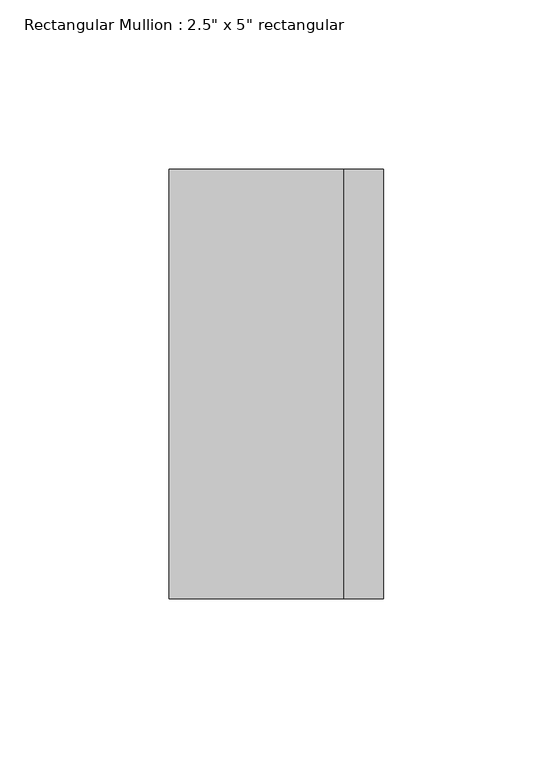
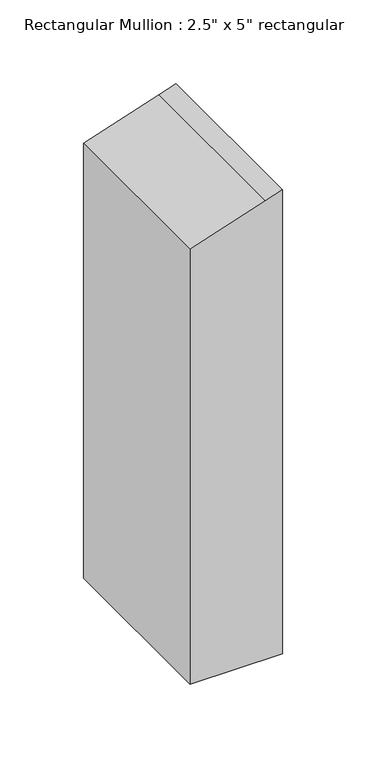
"""IFC4 building model written with IfcOpenShell, lengths in millimetres: member geometry."""

from ifc_helpers import new_model, si_unit, frame, origin, place, context, project, spatial, polyline, outline, extrude, source, transform, mapped, element, save


def member_4c11d242(model_context):
    return source(origin(), model_context, "Body", "SweptSolid", [
        extrude(outline(polyline([(-56.3515438, 31.75), (-60.2413894, 20.0804631), (-77.5182105, -31.75), (-394.1459231, -31.75), (-394.1459231, 31.75), (-56.3515438, 31.75)])), frame((0.0, -63.5, 0.0), z_axis=(0.0, 1.0, 0.0), x_axis=(0.0, 0.0, 1.0)), (0.0, 0.0, 1.0), 127.0),
    ])


if __name__ == "__main__":
    model = new_model("IFC4")
    model_context = context("Model", 3, world=origin())
    ifc_project = project(units=[si_unit("LENGTHUNIT", "METRE", prefix="MILLI")], contexts=[model_context])
    site = spatial("IfcSite", under=ifc_project)
    building = spatial("IfcBuilding", under=site)
    placement = place(None, origin())
    member_shape = member_4c11d242(model_context)
    element("IfcMember", 1, ObjectType="Rectangular Mullion : 2.5\" x 5\" rectangular", at=placement, inside=building, context=model_context, shape_type="MappedRepresentation", body=[
        mapped(member_shape, transform((0.0, 0.0, 0.0), x_axis=(1.0, 0.0, 0.0), y_axis=(0.0, 1.0, 0.0), z_axis=(0.0, 0.0, 1.0))),
    ])
    save(model, "model.ifc")

# Revit data of these elements
# Type "Rectangular Mullion : 2.5\" x 5\" rectangular"
#   built-in parameter 1007304 = 0.416667 (stored number, unit not read)
#   built-in parameter 1007301 = 0.104167 (stored number, unit not read)
#   built-in parameter 1007300 = 0.104167 (stored number, unit not read)
# Element 1 (IfcMember, "Rectangular Mullion : 2.5\" x 5\" rectangular")
#   Materials on its faces: "Metal - Aluminum"
# Materials
#   "Metal - Aluminum": class "Metal", colour RGB 140 140 140, transparency 0
